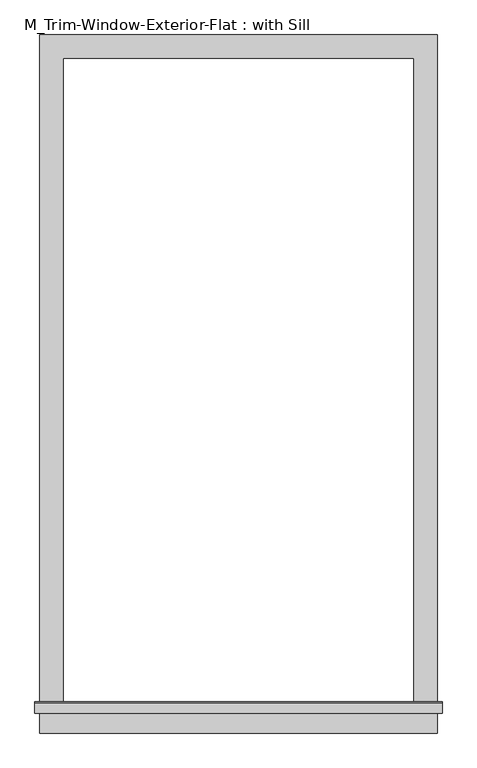
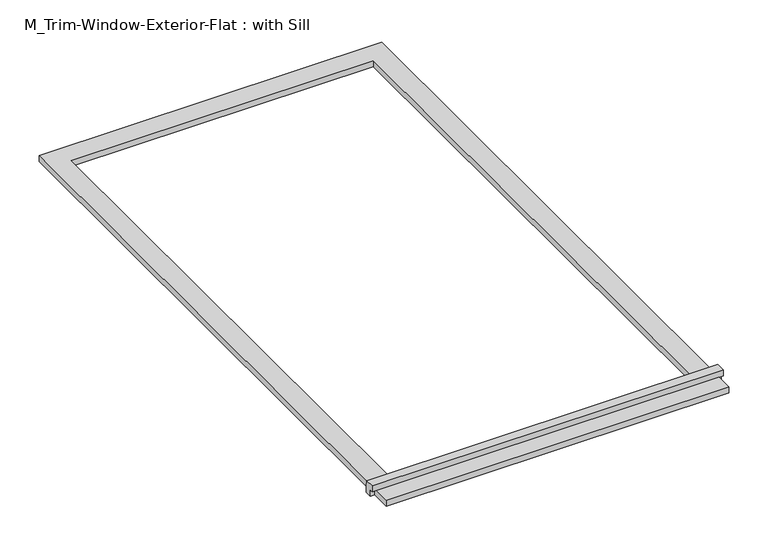
"""IFC4 building model written with IfcOpenShell, lengths in millimetres: proxy geometry, M_Trim-Window-Exterior-Flat : with Sill."""

import ifcopenshell
import ifcopenshell.guid

model = None  # the IFC model being written
_history = None  # IfcOwnerHistory: only IFC2X3 demands one
_inside = {}  # id of a spatial element -> (the spatial element, [elements in it])
_under = {}  # id of a project, library or spatial element -> (it, [spatial elements below it])
_declared = {}  # id of a project -> (the project, [libraries it declares])
_typed = {}  # id of a type object -> (the type object, [elements of that type])
_made_of = {}  # id of a material, layer set ... -> (it, [elements and type objects made of it])


def new_model(schema):
    """Start an empty IFC model of exactly this schema.

    Asked for "IFC4X3", IfcOpenShell would pick the latest addendum, in which some entities
    have other attributes; the version numbers below select the first issue.
    IFC2X3 requires an IfcOwnerHistory on every rooted entity: one is made here for all.
    """
    global model, _history
    if schema == "IFC4X3":
        model = ifcopenshell.file(schema_version=(4, 3, 0, 0))
    else:
        model = ifcopenshell.file(schema=schema)
    _inside.clear()
    _under.clear()
    _declared.clear()
    _typed.clear()
    _made_of.clear()
    _history = None
    if model.schema == "IFC2X3":
        org = make("IfcOrganization", Name="unknown")
        user = make(
            "IfcPersonAndOrganization",
            ThePerson=make("IfcPerson", FamilyName="unknown"),
            TheOrganization=org,
        )
        app = make(
            "IfcApplication",
            ApplicationDeveloper=org,
            Version="unknown",
            ApplicationFullName="unknown",
            ApplicationIdentifier="unknown",
        )
        _history = make(
            "IfcOwnerHistory",
            OwningUser=user,
            OwningApplication=app,
            ChangeAction="ADDED",
            CreationDate=0,
        )
    return model


def make(cls, **values):
    """One entity of the class cls with the attributes given. An attribute that is None is left unset."""
    return model.create_entity(
        cls, **{name: value for name, value in values.items() if value is not None}
    )


def rooted(cls, **values):
    """An entity with a GlobalId (a new one), such as an element, a storey or a relation."""
    return make(cls, GlobalId=ifcopenshell.guid.new(), OwnerHistory=_history, **values)


def si_unit(unit_type, name, prefix=None):
    """IfcSIUnit, for example si_unit("LENGTHUNIT", "METRE", prefix="MILLI")."""
    return make("IfcSIUnit", UnitType=unit_type, Prefix=prefix, Name=name)


def assignment(units):
    """IfcUnitAssignment: the units of a project."""
    return None if units is None else make("IfcUnitAssignment", Units=units)


def point(xyz):
    """IfcCartesianPoint."""
    return None if xyz is None else make("IfcCartesianPoint", Coordinates=xyz)


def direction(xyz):
    """IfcDirection."""
    return None if xyz is None else make("IfcDirection", DirectionRatios=xyz)


def frame(location, z_axis=None, x_axis=None):
    """IfcAxis2Placement3D, a coordinate frame: its origin and axes. An axis left out is left unset."""
    return make(
        "IfcAxis2Placement3D",
        Location=point(location),
        Axis=direction(z_axis),
        RefDirection=direction(x_axis),
    )


def origin():
    """The frame at (0, 0, 0) with its axes left unset."""
    return frame((0.0, 0.0, 0.0))


def origin_with_axes():
    """The frame at (0, 0, 0) with the z axis (0, 0, 1) and the x axis (1, 0, 0) written out."""
    return frame((0.0, 0.0, 0.0), z_axis=(0.0, 0.0, 1.0), x_axis=(1.0, 0.0, 0.0))


def place(relative_to, where):
    """IfcLocalPlacement: puts the frame where relative to a parent placement (None: the world)."""
    return make(
        "IfcLocalPlacement", PlacementRelTo=relative_to, RelativePlacement=where
    )


def context(
    kind, dimensions, precision=None, world=None, true_north=None, identifier=None
):
    """IfcGeometricRepresentationContext, for example the 3D "Model" context."""
    return make(
        "IfcGeometricRepresentationContext",
        ContextIdentifier=identifier,
        ContextType=kind,
        CoordinateSpaceDimension=dimensions,
        Precision=precision,
        WorldCoordinateSystem=world,
        TrueNorth=true_north,
    )


def project(units=None, contexts=None):
    """IfcProject with its units and contexts."""
    return rooted(
        "IfcProject",
        Name="project",
        RepresentationContexts=contexts,
        UnitsInContext=assignment(units),
    )


def spatial(cls, under=None, at=None, **own):
    """A site, building, storey or space (cls), placed at a placement, below another one or the project."""
    s = rooted(cls, ObjectPlacement=at, **own)
    if under is not None:
        _under.setdefault(under.id(), (under, []))[1].append(s)
    return s


def polyline(points):
    """IfcPolyline through the points."""
    return make("IfcPolyline", Points=[point(p) for p in points])


def outline(outer, holes=None, kind="AREA"):
    """IfcArbitraryClosedProfileDef: a profile drawn as a closed curve; with holes, ...WithVoids."""
    if holes is None:
        return make("IfcArbitraryClosedProfileDef", ProfileType=kind, OuterCurve=outer)
    return make(
        "IfcArbitraryProfileDefWithVoids",
        ProfileType=kind,
        OuterCurve=outer,
        InnerCurves=holes,
    )


def extrude(swept, where, along, depth):
    """IfcExtrudedAreaSolid: the profile swept, set in the frame where, extruded along a direction by depth."""
    return make(
        "IfcExtrudedAreaSolid",
        SweptArea=swept,
        Position=where,
        ExtrudedDirection=direction(along),
        Depth=depth,
    )


def shape(context_of_items, identifier, shape_type, items):
    """IfcShapeRepresentation: the items that make up one representation, for example the "Body"."""
    return make(
        "IfcShapeRepresentation",
        ContextOfItems=context_of_items,
        RepresentationIdentifier=identifier,
        RepresentationType=shape_type,
        Items=items,
    )


def source(mapping_origin, context_of_items, identifier, shape_type, items):
    """IfcRepresentationMap: a shape defined once, which mapped items show again and again."""
    return make(
        "IfcRepresentationMap",
        MappingOrigin=mapping_origin,
        MappedRepresentation=shape(context_of_items, identifier, shape_type, items),
    )


def transform(
    local_origin,
    x_axis=None,
    y_axis=None,
    z_axis=None,
    scale=None,
    scale2=None,
    scale3=None,
    uniform=True,
):
    """IfcCartesianTransformationOperator3D, or its non-uniform kind. x_axis, y_axis, z_axis: its Axis1, 2, 3."""
    if uniform:
        return make(
            "IfcCartesianTransformationOperator3D",
            Axis1=direction(x_axis),
            Axis2=direction(y_axis),
            LocalOrigin=point(local_origin),
            Scale=scale,
            Axis3=direction(z_axis),
        )
    return make(
        "IfcCartesianTransformationOperator3DnonUniform",
        Axis1=direction(x_axis),
        Axis2=direction(y_axis),
        LocalOrigin=point(local_origin),
        Scale=scale,
        Axis3=direction(z_axis),
        Scale2=scale2,
        Scale3=scale3,
    )


def mapped(mapping_source, mapping_target):
    """IfcMappedItem: shows the shape of a source again, moved by a transform."""
    return make(
        "IfcMappedItem", MappingSource=mapping_source, MappingTarget=mapping_target
    )


def made_of(thing, what):
    """Note that an element or type object is made of a material, layer set ...; save() writes the relation."""
    if what is not None:
        _made_of.setdefault(what.id(), (what, []))[1].append(thing)
    return thing


def element(
    cls,
    number,
    at=None,
    inside=None,
    cuts=None,
    type_object=None,
    material=None,
    context=None,
    identifier="Body",
    shape_type=None,
    held_by="IfcProductDefinitionShape",
    body=None,
    shapes=None,
    **own,
):
    """One element of the class cls, such as IfcWall. Its Tag is "e" and its number.

    at: its placement. inside: the storey or other place that contains it. cuts: it is an
    opening in that element (IfcRelVoidsElement). A single representation is given by context,
    identifier, shape_type and body (its items); several are given by shapes. held_by: the class
    of the entity that holds the representations. save() writes the other relations.
    """
    e = rooted(cls, Tag="e%d" % number, ObjectPlacement=at, **own)
    if body is not None:
        shapes = [shape(context, identifier, shape_type, body)]
    if shapes is not None:
        e.Representation = make(held_by, Representations=shapes)
    if inside is not None:
        _inside.setdefault(inside.id(), (inside, []))[1].append(e)
    if cuts is not None:
        rooted(
            "IfcRelVoidsElement", RelatingBuildingElement=cuts, RelatedOpeningElement=e
        )
    if type_object is not None:
        _typed.setdefault(type_object.id(), (type_object, []))[1].append(e)
    return made_of(e, material)


def aggregate(whole, parts):
    """IfcRelAggregates: a whole, such as a stair, and the parts it consists of."""
    return rooted("IfcRelAggregates", RelatingObject=whole, RelatedObjects=parts)


def save(model, path):
    """Write the relations noted so far, then the file.

    IfcRelAggregates (storeys below a building ...), IfcRelContainedInSpatialStructure (elements
    in a storey), IfcRelDefinesByType, IfcRelAssociatesMaterial and IfcRelDeclares: one each for
    every whole, place, type object, material and project.
    """
    for whole, parts in _under.values():
        aggregate(whole, parts)
    for where, things in _inside.values():
        rooted(
            "IfcRelContainedInSpatialStructure",
            RelatedElements=things,
            RelatingStructure=where,
        )
    for kind, things in _typed.values():
        rooted("IfcRelDefinesByType", RelatedObjects=things, RelatingType=kind)
    for what, things in _made_of.values():
        rooted("IfcRelAssociatesMaterial", RelatedObjects=things, RelatingMaterial=what)
    for by, libraries in _declared.values():
        rooted("IfcRelDeclares", RelatingContext=by, RelatedDefinitions=libraries)
    model.write(path)


def m_trim_window_exterior_flat_with_sill_09d1e46a(model_context):
    return source(origin(), model_context, "Body", "SweptSolid", [
        extrude(outline(polyline([(510.0, -1670.4323709), (510.0, -1730.4323709), (-510.0, -1730.4323709), (-510.0, -1670.4323709), (510.0, -1670.4323709)])), origin_with_axes(), (0.0, 0.0, 1.0), 19.05),
        extrude(outline(polyline([(-1680.0, 38.1), (-1652.4580645, 38.1), (-1650.0, 19.05), (-1650.0, 0.0), (-1670.4323709, 0.0), (-1670.4323709, 19.05), (-1680.0, 19.05), (-1680.0, 38.1)])), frame((-522.7, 0.0, 0.0), z_axis=(1.0, 0.0, 0.0), x_axis=(0.0, 1.0, 0.0)), (0.0, 0.0, 1.0), 1045.4),
        extrude(outline(polyline([(-510.0, 60.0), (510.0, 60.0), (510.0, -1650.0), (450.0, -1650.0), (450.0, 0.0), (-450.0, 0.0), (-450.0, -1650.0), (-510.0, -1650.0), (-510.0, 60.0)])), origin_with_axes(), (0.0, 0.0, 1.0), 19.05),
    ])


if __name__ == "__main__":
    model = new_model("IFC4")
    model_context = context("Model", 3, world=origin())
    ifc_project = project(units=[si_unit("LENGTHUNIT", "METRE", prefix="MILLI")], contexts=[model_context])
    site = spatial("IfcSite", under=ifc_project)
    building = spatial("IfcBuilding", under=site)
    placement = place(None, origin())
    m_trim_window_exterior_flat_with_sill_shape = m_trim_window_exterior_flat_with_sill_09d1e46a(model_context)
    element("IfcBuildingElementProxy", 1, Name="M_Trim-Window-Exterior-Flat : with Sill", ObjectType="M_Trim-Window-Exterior-Flat : with Sill", at=placement, inside=building, context=model_context, shape_type="MappedRepresentation", body=[
        mapped(m_trim_window_exterior_flat_with_sill_shape, transform((0.0, 0.0, 0.0), x_axis=(1.0, 0.0, 0.0), y_axis=(0.0, 1.0, 0.0), z_axis=(0.0, 0.0, 1.0))),
    ])
    save(model, "model.ifc")

# Revit data of these elements
# Type "M_Trim-Window-Exterior-Flat : with Sill"
#   Trim Width = 60 mm
#   Trim Thickness_Picture Frame = 30 mm
#   Trim Thickness_with Sill = 19.05 mm
#   Sill Thickness = 30 mm
#   Opening Width [instance default] = 600 mm
#   Opening Height [instance default] = 900 mm
#   Default Elevation = 1200 mm
#   Sill = yes
#   Picture Frame = no
#   Trim Material [instance default] = none
# Element 1 (IfcBuildingElementProxy, "M_Trim-Window-Exterior-Flat : with Sill")
#   Opening Width = 900 mm
#   Opening Height = 1650 mm
#   Trim Material = Clad - White
#   Materials on its faces: "Clad - White"
# Materials
#   "Clad - White": class "Wood", colour RGB 245 245 243, transparency 0, Cost = 0
